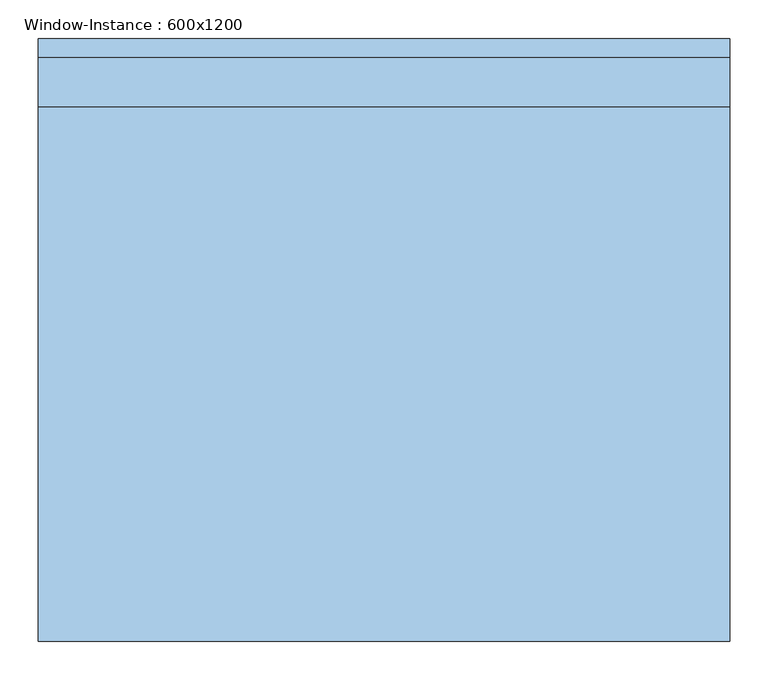
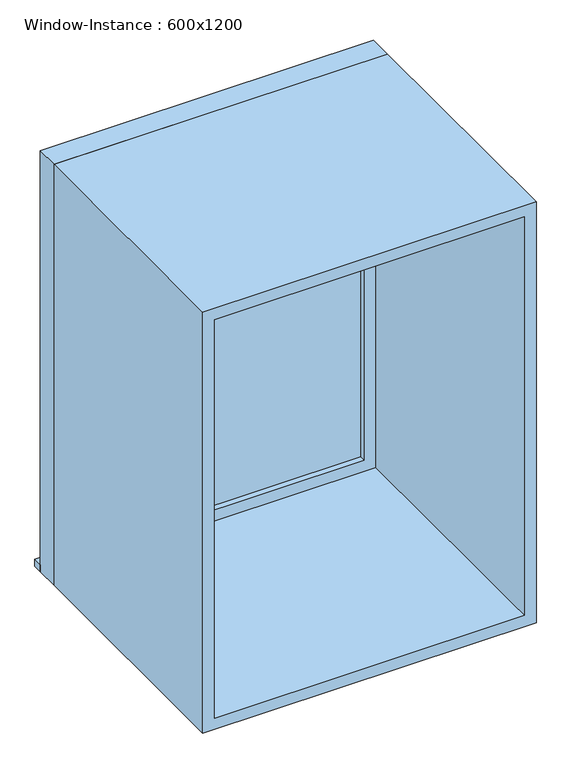
"""IFC4 building model written with IfcOpenShell, lengths in millimetres: window geometry, Window-Instance : 600x1200."""

from ifc_helpers import new_model, si_unit, frame, origin, place, context, project, spatial, polyline, outline, extrude, source, transform, mapped, element, save


def window_instance_600x1200_3a897e98(model_context):
    return source(origin(), model_context, "Body", "SweptSolid", [
        extrude(outline(polyline([(-488.1, 405.4), (411.9, 405.4), (411.9, 380.0), (-488.1, 380.0), (-488.1, 405.4)])), frame((0.0, 0.0, 900.0), z_axis=(0.0, 0.0, 1.0), x_axis=(1.0, 0.0, 0.0)), (0.0, 0.0, 1.0), 19.05),
        extrude(outline(polyline([(348.4, 331.425), (-424.6, 331.425), (-424.6, 344.125), (348.4, 344.125), (348.4, 331.425)])), frame((0.0, 0.0, 963.5), z_axis=(0.0, 0.0, 1.0), x_axis=(1.0, 0.0, 0.0)), (0.0, 0.0, 1.0), 1073.0),
        extrude(outline(polyline([(2080.95, -469.05), (919.05, -469.05), (919.05, 392.85), (2080.95, 392.85), (2080.95, -469.05)]), holes=[polyline([(2036.5, -424.6), (2036.5, 348.4), (963.5, 348.4), (963.5, -424.6), (2036.5, -424.6)])]), frame((0.0, 315.55, 0.0), z_axis=(0.0, 1.0, 0.0), x_axis=(0.0, 0.0, 1.0)), (0.0, 0.0, 1.0), 44.45),
        extrude(outline(polyline([(2100.0, -488.1), (900.0, -488.1), (900.0, 411.9), (2100.0, 411.9), (2100.0, -488.1)]), holes=[polyline([(2068.25, -456.35), (2068.25, 380.15), (931.75, 380.15), (931.75, -456.35), (2068.25, -456.35)])]), frame((0.0, -380.0, 0.0), z_axis=(0.0, 1.0, 0.0), x_axis=(0.0, 0.0, 1.0)), (0.0, 0.0, 1.0), 695.55),
        extrude(outline(polyline([(2100.0, 411.9), (2100.0, -488.1), (900.0, -488.1), (900.0, 411.9), (2100.0, 411.9)]), holes=[polyline([(2080.95, 392.85), (919.05, 392.85), (919.05, -469.05), (2080.95, -469.05), (2080.95, 392.85)])]), frame((0.0, 315.55, 0.0), z_axis=(0.0, 1.0, 0.0), x_axis=(0.0, 0.0, 1.0)), (0.0, 0.0, 1.0), 64.45),
    ])


if __name__ == "__main__":
    model = new_model("IFC4")
    model_context = context("Model", 3, world=origin())
    ifc_project = project(units=[si_unit("LENGTHUNIT", "METRE", prefix="MILLI")], contexts=[model_context])
    site = spatial("IfcSite", under=ifc_project)
    building = spatial("IfcBuilding", under=site)
    placement = place(None, origin())
    window_instance_600x1200_shape = window_instance_600x1200_3a897e98(model_context)
    element("IfcWindow", 1, ObjectType="Window-Instance : 600x1200", at=placement, inside=building, context=model_context, shape_type="MappedRepresentation", body=[
        mapped(window_instance_600x1200_shape, transform((0.0, 0.0, 0.0), x_axis=(1.0, 0.0, 0.0), y_axis=(0.0, 1.0, 0.0), z_axis=(0.0, 0.0, 1.0))),
    ])
    save(model, "model.ifc")

# Revit data of these elements
# Type "Window-Instance : 600x1200"
#   Type Mark = "7"
#   Construction Type Id = "GSP4R"
#   Assembly Code = "B2020100"
#   Analytic Construction = "1/8 in Pilkington single glazing"
#   Visual Light Transmittance = 0.9
#   Thermal Resistance (R) = 0.149095 (m²·K)/W
#   Solar Heat Gain Coefficient = 0.86
#   Heat Transfer Coefficient (U) = 6.70716 W/(m²·K)
#   Height [instance default] = 1200 mm
#   Default Sill Height = 900 mm
#   Width [instance default] = 600 mm
#   Window Inset = 20 mm
#   Glass Pane Material = WW-EC-GL-Storefront
#   Sash Material = WW-EC-RGB-White
#   Wall Closure = (empty or 0)
# Element 1 (IfcWindow, "Window-Instance : 600x1200")
#   Width = 900 mm
#   Materials on its faces: "WW-EC-RGB-White", "WW-EC-GL-Storefront"
# Materials
#   "WW-EC-GL-Storefront": class "Glass", colour RGB 236 240 239, transparency 0.85, Description = "Storefront Glass", Cost = 0
#   "WW-EC-RGB-White": class "Generic", colour RGB 255 255 255, transparency 0, Comments = "If region requests off-white, swith asset color to RGB 231-228-220", Description = "Generic Color", Cost = 0
